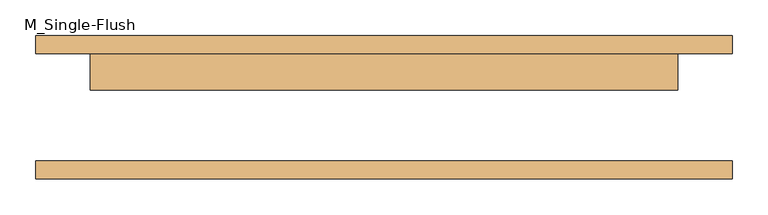
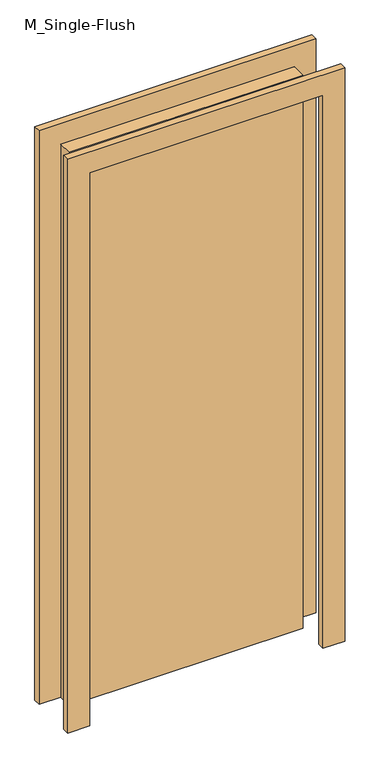
"""IFC4 building model written with IfcOpenShell, lengths in millimetres: door geometry, M_Single-Flush : iç kapı 1."""

from ifc_helpers import new_model, si_unit, frame, origin, origin_with_axes, place, context, project, spatial, polyline, outline, extrude, source, transform, mapped, element, save


def m_single_flush_16974dc2(model_context):
    return source(origin(), model_context, "Body", "SweptSolid", [
        extrude(outline(polyline([(2126.0, -486.0), (0.0, -486.0), (0.0, -410.0), (2050.0, -410.0), (2050.0, 410.0), (0.0, 410.0), (0.0, 486.0), (2126.0, 486.0), (2126.0, -486.0)])), frame((0.0, 75.0, 0.0), z_axis=(0.0, 1.0, 0.0), x_axis=(0.0, 0.0, 1.0)), (0.0, 0.0, 1.0), 25.0),
        extrude(outline(polyline([(2126.0, 486.0), (2126.0, -486.0), (0.0, -486.0), (0.0, -410.0), (2050.0, -410.0), (2050.0, 410.0), (0.0, 410.0), (0.0, 486.0), (2126.0, 486.0)])), frame((0.0, -100.0, 0.0), z_axis=(0.0, 1.0, 0.0), x_axis=(0.0, 0.0, 1.0)), (0.0, 0.0, 1.0), 25.0),
        extrude(outline(polyline([(410.0, 24.0), (-410.0, 24.0), (-410.0, 75.0), (410.0, 75.0), (410.0, 24.0)])), origin_with_axes(), (0.0, 0.0, 1.0), 2050.0),
    ])


if __name__ == "__main__":
    model = new_model("IFC4")
    model_context = context("Model", 3, world=origin())
    ifc_project = project(units=[si_unit("LENGTHUNIT", "METRE", prefix="MILLI")], contexts=[model_context])
    site = spatial("IfcSite", under=ifc_project)
    building = spatial("IfcBuilding", under=site)
    placement = place(None, origin())
    m_single_flush_shape = m_single_flush_16974dc2(model_context)
    element("IfcDoor", 1, ObjectType="M_Single-Flush : iç kapı 1", at=placement, inside=building, context=model_context, shape_type="MappedRepresentation", body=[
        mapped(m_single_flush_shape, transform((0.0, 0.0, 0.0), x_axis=(1.0, 0.0, 0.0), y_axis=(0.0, 1.0, 0.0), z_axis=(0.0, 0.0, 1.0))),
    ])
    save(model, "model.ifc")

# Revit data of these elements
# Type "M_Single-Flush : iç kapı 1"
#   Type Mark = "24"
#   Construction Type Id = "MDOOR"
#   Analytic Construction = "Metal"
#   Thickness = 5.1 cm
#   Thermal Resistance (R) = 0.270117 (m²·K)/W
#   Heat Transfer Coefficient (U) = 3.7021 W/(m²·K)
#   Height = 205 cm
#   Trim Projection Ext = 2.5 cm
#   Trim Projection Int = 2.5 cm
#   Trim Width = 7.6 cm
#   Width = 82 cm
#   Define Thermal Properties by = 1
#   Door Material = Door - Panel
#   Frame Material = Door - Frame
#   Visual Light Transmittance = 0
#   Solar Heat Gain Coefficient = 0
#   Function = (empty or 0)
#   Wall Closure = (empty or 0)
# Element 1 (IfcDoor, "M_Single-Flush : iç kapı 1")
#   Materials on its faces: "Door - Frame", "Door - Panel"
# Materials
#   "Door - Panel": class "Wood", colour RGB 210 159 95, transparency 0, Cost = 0
#   "Door - Frame": class "Miscellaneous", colour RGB 118 70 51, transparency 0, Cost = 0
